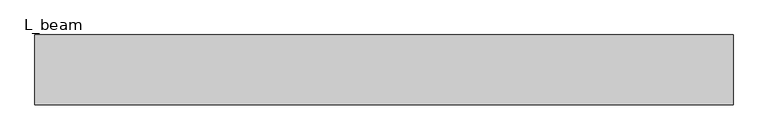
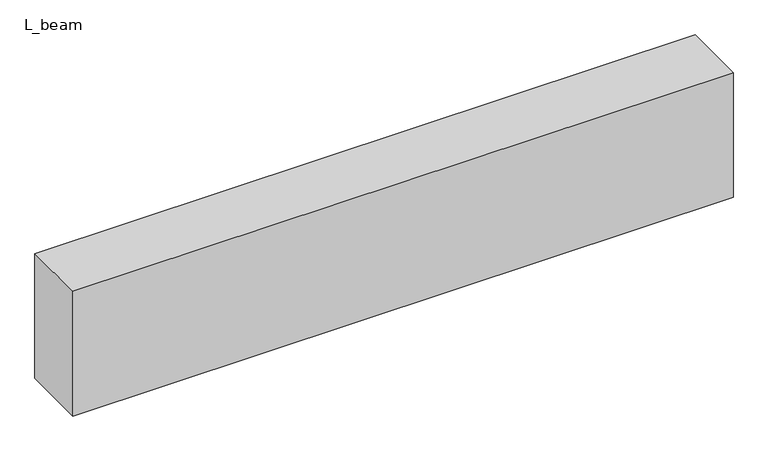
"""IFC4 building model written with IfcOpenShell, lengths in millimetres: beam geometry, 混凝土 - 矩形梁 : L_beam."""

from ifc_helpers import new_model, si_unit, frame, origin, place, context, project, spatial, polyline, outline, extrude, source, transform, mapped, element, save


def l_beam_6aa05230(model_context):
    return source(origin(), model_context, "Body", "SweptSolid", [
        extrude(outline(polyline([(1501.5, 150.0), (1501.5, -150.0), (-1501.5, -150.0), (-1501.5, 150.0), (1501.5, 150.0)])), frame((0.0, 0.0, -300.0), z_axis=(0.0, 0.0, 1.0), x_axis=(1.0, 0.0, 0.0)), (0.0, 0.0, 1.0), 600.0),
    ])


if __name__ == "__main__":
    model = new_model("IFC4")
    model_context = context("Model", 3, world=origin())
    ifc_project = project(units=[si_unit("LENGTHUNIT", "METRE", prefix="MILLI")], contexts=[model_context])
    site = spatial("IfcSite", under=ifc_project)
    building = spatial("IfcBuilding", under=site)
    placement = place(None, origin())
    l_beam_shape = l_beam_6aa05230(model_context)
    element("IfcBeam", 1, ObjectType="混凝土 - 矩形梁 : L_beam", at=placement, inside=building, context=model_context, shape_type="MappedRepresentation", body=[
        mapped(l_beam_shape, transform((0.0, 0.0, 0.0), x_axis=(1.0, 0.0, 0.0), y_axis=(0.0, 1.0, 0.0), z_axis=(0.0, 0.0, 1.0))),
    ])
    save(model, "model.ifc")

# Revit data of these elements
# Type "混凝土 - 矩形梁 : L_beam"
#   Length [instance default] = 1524 mm
#   b = 300 mm
#   h = 600 mm
#   Structural Material [instance default] = none
#   Assembly Code = ""
